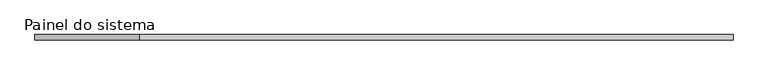
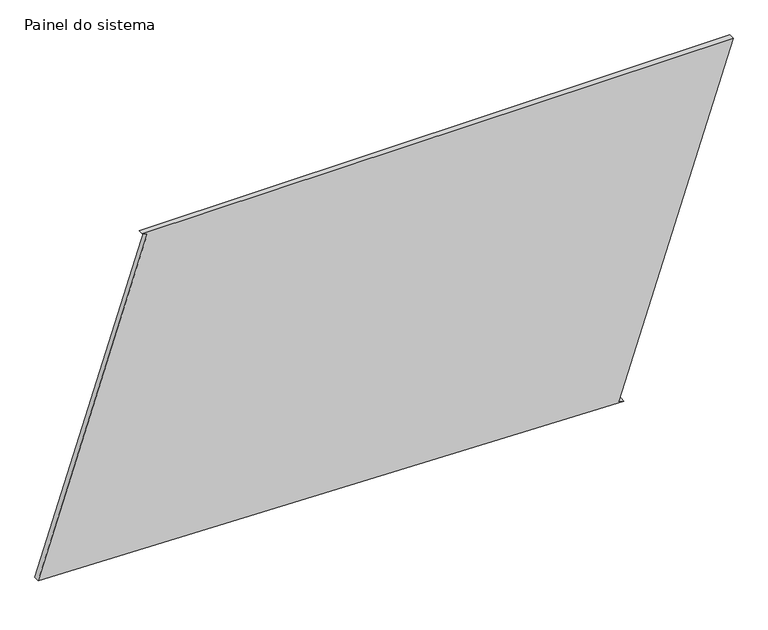
"""IFC4 building model written with IfcOpenShell, lengths in millimetres: plate geometry, Painel do sistema : Envidraçado."""

from ifc_helpers import new_model, si_unit, frame, origin, place, context, project, spatial, polyline, outline, extrude, source, transform, mapped, element, save


def painel_do_sistema_a31b9cd7(model_context):
    return source(origin(), model_context, "Body", "SweptSolid", [
        extrude(outline(polyline([(0.0, 1082.7302621), (7.8961296, 1059.0099936), (1570.25148, 1579.0951856), (1570.25148, -1105.9808078), (1562.3553504, -1082.2605393), (69.8455081, -1579.0951856), (0.0, 1082.7302621)])), frame((0.0, 24.5, 0.0), z_axis=(0.0, 1.0, 0.0), x_axis=(0.0, 0.0, 1.0)), (0.0, 0.0, 1.0), 25.0),
    ])


if __name__ == "__main__":
    model = new_model("IFC4")
    model_context = context("Model", 3, world=origin())
    ifc_project = project(units=[si_unit("LENGTHUNIT", "METRE", prefix="MILLI")], contexts=[model_context])
    site = spatial("IfcSite", under=ifc_project)
    building = spatial("IfcBuilding", under=site)
    placement = place(None, origin())
    painel_do_sistema_shape = painel_do_sistema_a31b9cd7(model_context)
    element("IfcPlate", 1, ObjectType="Painel do sistema : Envidraçado", at=placement, inside=building, context=model_context, shape_type="MappedRepresentation", body=[
        mapped(painel_do_sistema_shape, transform((0.0, 0.0, 0.0), x_axis=(1.0, 0.0, 0.0), y_axis=(0.0, 1.0, 0.0), z_axis=(0.0, 0.0, 1.0))),
    ])
    save(model, "model.ifc")

# Revit data of these elements
# Type "Painel do sistema : Envidraçado"
#   Construction Type Id = "GSP4R"
#   Analytic Construction = "Vidraça única Pilkington 1/8 pol"
#   Visual Light Transmittance = 0.9
#   Solar Heat Gain Coefficient = 0.86
#   Heat Transfer Coefficient (U) = 6.7069 W/(m²·K)
# Element 1 (IfcPlate, "Painel do sistema : Envidraçado")
#   Materials on its faces: "Vidro"
# Materials
#   "Vidro": class "Vidro", colour RGB 0 128 192, transparency 0.9, Description = "Vidro de sílica", Cost = 0
